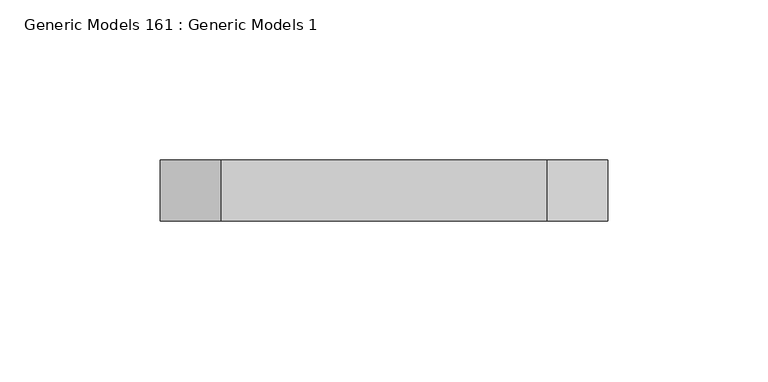
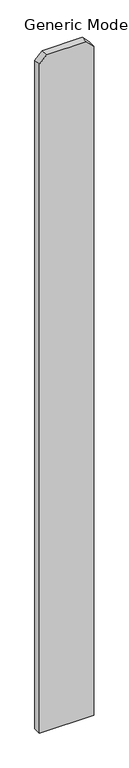
"""IFC4 building model written with IfcOpenShell, lengths in millimetres: proxy geometry, Generic Models 161 : Generic Models 1."""

from ifc_helpers import new_model, si_unit, frame, origin, place, context, project, spatial, polyline, outline, extrude, source, transform, mapped, element, save


def generic_models_161_generic_models_1_936b907a(model_context):
    return source(origin(), model_context, "Body", "SweptSolid", [
        extrude(outline(polyline([(76.2, -250267.7875), (1885.95, -250267.7875), (1905.0, -250286.8375), (1905.0, -250388.4375), (1885.95, -250407.4875), (76.2, -250407.4875), (76.2, -250267.7875)])), frame((0.0, 547.6875, 0.0), z_axis=(0.0, 1.0, 0.0), x_axis=(0.0, 0.0, 1.0)), (0.0, 0.0, 1.0), 19.05),
    ])


if __name__ == "__main__":
    model = new_model("IFC4")
    model_context = context("Model", 3, world=origin())
    ifc_project = project(units=[si_unit("LENGTHUNIT", "METRE", prefix="MILLI")], contexts=[model_context])
    site = spatial("IfcSite", under=ifc_project)
    building = spatial("IfcBuilding", under=site)
    placement = place(None, origin())
    generic_models_161_generic_models_1_shape = generic_models_161_generic_models_1_936b907a(model_context)
    element("IfcBuildingElementProxy", 1, Name="Generic Models 161 : Generic Models 1", ObjectType="Generic Models 161 : Generic Models 1", at=placement, inside=building, context=model_context, shape_type="MappedRepresentation", body=[
        mapped(generic_models_161_generic_models_1_shape, transform((0.0, 0.0, 0.0), x_axis=(1.0, 0.0, 0.0), y_axis=(0.0, 1.0, 0.0), z_axis=(0.0, 0.0, 1.0))),
    ])
    save(model, "model.ifc")

# Revit data of these elements
# Element 1 (IfcBuildingElementProxy, "Generic Models 161 : Generic Models 1")
#   Materials on its faces: "VERTICAL 1X6 CEDAR PLANKS W/ CLEAR WOOD SEALER"
# Materials
#   "VERTICAL 1X6 CEDAR PLANKS W/ CLEAR WOOD SEALER": class "Wood", colour RGB 234 198 147, transparency 0, Description = "Pinus Echinata", Cost = 0
